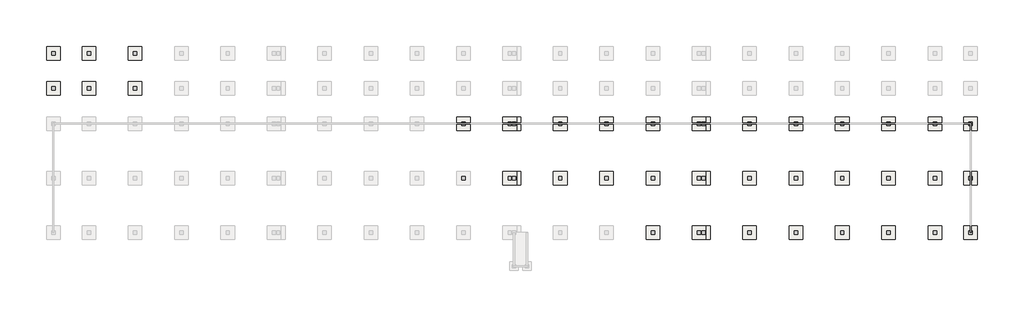
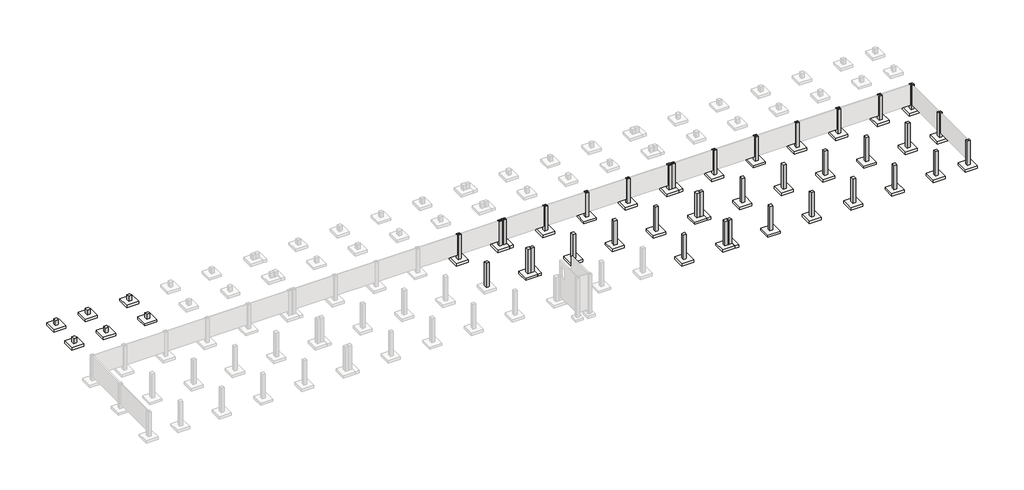
# Not in any storey, part 2 of 3: 43 columns, 42 slabs.
"""IFC4 building model written with IfcOpenShell, lengths in millimetres."""

import ifcopenshell
import ifcopenshell.guid

model = None  # the IFC model being written
_history = None  # IfcOwnerHistory: only IFC2X3 demands one
_inside = {}  # id of a spatial element -> (the spatial element, [elements in it])
_under = {}  # id of a project, library or spatial element -> (it, [spatial elements below it])
_declared = {}  # id of a project -> (the project, [libraries it declares])
_typed = {}  # id of a type object -> (the type object, [elements of that type])
_made_of = {}  # id of a material, layer set ... -> (it, [elements and type objects made of it])


def new_model(schema):
    """Start an empty IFC model of exactly this schema.

    Asked for "IFC4X3", IfcOpenShell would pick the latest addendum, in which some entities
    have other attributes; the version numbers below select the first issue.
    IFC2X3 requires an IfcOwnerHistory on every rooted entity: one is made here for all.
    """
    global model, _history
    if schema == "IFC4X3":
        model = ifcopenshell.file(schema_version=(4, 3, 0, 0))
    else:
        model = ifcopenshell.file(schema=schema)
    _inside.clear()
    _under.clear()
    _declared.clear()
    _typed.clear()
    _made_of.clear()
    _history = None
    if model.schema == "IFC2X3":
        org = make("IfcOrganization", Name="unknown")
        user = make(
            "IfcPersonAndOrganization",
            ThePerson=make("IfcPerson", FamilyName="unknown"),
            TheOrganization=org,
        )
        app = make(
            "IfcApplication",
            ApplicationDeveloper=org,
            Version="unknown",
            ApplicationFullName="unknown",
            ApplicationIdentifier="unknown",
        )
        _history = make(
            "IfcOwnerHistory",
            OwningUser=user,
            OwningApplication=app,
            ChangeAction="ADDED",
            CreationDate=0,
        )
    return model


def make(cls, **values):
    """One entity of the class cls with the attributes given. An attribute that is None is left unset."""
    return model.create_entity(
        cls, **{name: value for name, value in values.items() if value is not None}
    )


def rooted(cls, **values):
    """An entity with a GlobalId (a new one), such as an element, a storey or a relation."""
    return make(cls, GlobalId=ifcopenshell.guid.new(), OwnerHistory=_history, **values)


def si_unit(unit_type, name, prefix=None):
    """IfcSIUnit, for example si_unit("LENGTHUNIT", "METRE", prefix="MILLI")."""
    return make("IfcSIUnit", UnitType=unit_type, Prefix=prefix, Name=name)


def assignment(units):
    """IfcUnitAssignment: the units of a project."""
    return None if units is None else make("IfcUnitAssignment", Units=units)


def point(xyz):
    """IfcCartesianPoint."""
    return None if xyz is None else make("IfcCartesianPoint", Coordinates=xyz)


def direction(xyz):
    """IfcDirection."""
    return None if xyz is None else make("IfcDirection", DirectionRatios=xyz)


def frame(location, z_axis=None, x_axis=None):
    """IfcAxis2Placement3D, a coordinate frame: its origin and axes. An axis left out is left unset."""
    return make(
        "IfcAxis2Placement3D",
        Location=point(location),
        Axis=direction(z_axis),
        RefDirection=direction(x_axis),
    )


def origin():
    """The frame at (0, 0, 0) with its axes left unset."""
    return frame((0.0, 0.0, 0.0))


def place(relative_to, where):
    """IfcLocalPlacement: puts the frame where relative to a parent placement (None: the world)."""
    return make(
        "IfcLocalPlacement", PlacementRelTo=relative_to, RelativePlacement=where
    )


def context(
    kind, dimensions, precision=None, world=None, true_north=None, identifier=None
):
    """IfcGeometricRepresentationContext, for example the 3D "Model" context."""
    return make(
        "IfcGeometricRepresentationContext",
        ContextIdentifier=identifier,
        ContextType=kind,
        CoordinateSpaceDimension=dimensions,
        Precision=precision,
        WorldCoordinateSystem=world,
        TrueNorth=true_north,
    )


def project(units=None, contexts=None):
    """IfcProject with its units and contexts."""
    return rooted(
        "IfcProject",
        Name="project",
        RepresentationContexts=contexts,
        UnitsInContext=assignment(units),
    )


def spatial(cls, under=None, at=None, **own):
    """A site, building, storey or space (cls), placed at a placement, below another one or the project."""
    s = rooted(cls, ObjectPlacement=at, **own)
    if under is not None:
        _under.setdefault(under.id(), (under, []))[1].append(s)
    return s


def polyline(points):
    """IfcPolyline through the points."""
    return make("IfcPolyline", Points=[point(p) for p in points])


def outline(outer, holes=None, kind="AREA"):
    """IfcArbitraryClosedProfileDef: a profile drawn as a closed curve; with holes, ...WithVoids."""
    if holes is None:
        return make("IfcArbitraryClosedProfileDef", ProfileType=kind, OuterCurve=outer)
    return make(
        "IfcArbitraryProfileDefWithVoids",
        ProfileType=kind,
        OuterCurve=outer,
        InnerCurves=holes,
    )


def extrude(swept, where, along, depth):
    """IfcExtrudedAreaSolid: the profile swept, set in the frame where, extruded along a direction by depth."""
    return make(
        "IfcExtrudedAreaSolid",
        SweptArea=swept,
        Position=where,
        ExtrudedDirection=direction(along),
        Depth=depth,
    )


def shape(context_of_items, identifier, shape_type, items):
    """IfcShapeRepresentation: the items that make up one representation, for example the "Body"."""
    return make(
        "IfcShapeRepresentation",
        ContextOfItems=context_of_items,
        RepresentationIdentifier=identifier,
        RepresentationType=shape_type,
        Items=items,
    )


def source(mapping_origin, context_of_items, identifier, shape_type, items):
    """IfcRepresentationMap: a shape defined once, which mapped items show again and again."""
    return make(
        "IfcRepresentationMap",
        MappingOrigin=mapping_origin,
        MappedRepresentation=shape(context_of_items, identifier, shape_type, items),
    )


def transform(
    local_origin,
    x_axis=None,
    y_axis=None,
    z_axis=None,
    scale=None,
    scale2=None,
    scale3=None,
    uniform=True,
):
    """IfcCartesianTransformationOperator3D, or its non-uniform kind. x_axis, y_axis, z_axis: its Axis1, 2, 3."""
    if uniform:
        return make(
            "IfcCartesianTransformationOperator3D",
            Axis1=direction(x_axis),
            Axis2=direction(y_axis),
            LocalOrigin=point(local_origin),
            Scale=scale,
            Axis3=direction(z_axis),
        )
    return make(
        "IfcCartesianTransformationOperator3DnonUniform",
        Axis1=direction(x_axis),
        Axis2=direction(y_axis),
        LocalOrigin=point(local_origin),
        Scale=scale,
        Axis3=direction(z_axis),
        Scale2=scale2,
        Scale3=scale3,
    )


def mapped(mapping_source, mapping_target):
    """IfcMappedItem: shows the shape of a source again, moved by a transform."""
    return make(
        "IfcMappedItem", MappingSource=mapping_source, MappingTarget=mapping_target
    )


def made_of(thing, what):
    """Note that an element or type object is made of a material, layer set ...; save() writes the relation."""
    if what is not None:
        _made_of.setdefault(what.id(), (what, []))[1].append(thing)
    return thing


def element(
    cls,
    number,
    at=None,
    inside=None,
    cuts=None,
    type_object=None,
    material=None,
    context=None,
    identifier="Body",
    shape_type=None,
    held_by="IfcProductDefinitionShape",
    body=None,
    shapes=None,
    **own,
):
    """One element of the class cls, such as IfcWall. Its Tag is "e" and its number.

    at: its placement. inside: the storey or other place that contains it. cuts: it is an
    opening in that element (IfcRelVoidsElement). A single representation is given by context,
    identifier, shape_type and body (its items); several are given by shapes. held_by: the class
    of the entity that holds the representations. save() writes the other relations.
    """
    e = rooted(cls, Tag="e%d" % number, ObjectPlacement=at, **own)
    if body is not None:
        shapes = [shape(context, identifier, shape_type, body)]
    if shapes is not None:
        e.Representation = make(held_by, Representations=shapes)
    if inside is not None:
        _inside.setdefault(inside.id(), (inside, []))[1].append(e)
    if cuts is not None:
        rooted(
            "IfcRelVoidsElement", RelatingBuildingElement=cuts, RelatedOpeningElement=e
        )
    if type_object is not None:
        _typed.setdefault(type_object.id(), (type_object, []))[1].append(e)
    return made_of(e, material)


def aggregate(whole, parts):
    """IfcRelAggregates: a whole, such as a stair, and the parts it consists of."""
    return rooted("IfcRelAggregates", RelatingObject=whole, RelatedObjects=parts)


def save(model, path):
    """Write the relations noted so far, then the file.

    IfcRelAggregates (storeys below a building ...), IfcRelContainedInSpatialStructure (elements
    in a storey), IfcRelDefinesByType, IfcRelAssociatesMaterial and IfcRelDeclares: one each for
    every whole, place, type object, material and project.
    """
    for whole, parts in _under.values():
        aggregate(whole, parts)
    for where, things in _inside.values():
        rooted(
            "IfcRelContainedInSpatialStructure",
            RelatedElements=things,
            RelatingStructure=where,
        )
    for kind, things in _typed.values():
        rooted("IfcRelDefinesByType", RelatedObjects=things, RelatingType=kind)
    for what, things in _made_of.values():
        rooted("IfcRelAssociatesMaterial", RelatedObjects=things, RelatingMaterial=what)
    for by, libraries in _declared.values():
        rooted("IfcRelDeclares", RelatingContext=by, RelatedDefinitions=libraries)
    model.write(path)


def foundation_rectangular_non_pile_5fe39465(model_context):
    return source(origin(), model_context, "Body", "SweptSolid", [
        extrude(outline(polyline([(1200.0, 1200.0), (1200.0, -1200.0), (-1200.0, -1200.0), (-1200.0, 1200.0), (1200.0, 1200.0)])), frame((0.0, 0.0, -500.0), z_axis=(0.0, 0.0, 1.0), x_axis=(1.0, 0.0, 0.0)), (0.0, 0.0, 1.0), 500.0),
    ])


model = new_model("IFC4")

# Units and contexts
model_context = context("Model", 3, world=origin())
ifc_project = project(units=[si_unit("LENGTHUNIT", "METRE", prefix="MILLI")], contexts=[model_context])

# Site, building
site = spatial("IfcSite", under=ifc_project)
building = spatial("IfcBuilding", under=site)

# Columns
placement = place(None, origin())
element("IfcColumn", 1, ObjectType="RC_Column_Rectangular : H_SC_AR_S15_UG PED_W600xL600_Bit_Anchor", at=placement, inside=building, context=model_context, shape_type="SweptSolid", body=[
    extrude(outline(polyline([(-4070.0, 549.5208589), (-4070.0, -50.4791411), (-4670.0, -50.4791411), (-4670.0, 549.5208589), (-4070.0, 549.5208589)])), frame((0.0, 0.0, -750.0381366), z_axis=(0.0, 0.0, 1.0), x_axis=(1.0, 0.0, 0.0)), (0.0, 0.0, 1.0), 1050.0),
])
element("IfcColumn", 2, ObjectType="RC_Column_Rectangular : H_SC_AR_S15_UG PED_W600xL600_Bit_Anchor", at=placement, inside=building, context=model_context, shape_type="SweptSolid", body=[
    extrude(outline(polyline([(2230.0, 549.5208589), (2230.0, -50.4791411), (1630.0, -50.4791411), (1630.0, 549.5208589), (2230.0, 549.5208589)])), frame((0.0, 0.0, -750.0381366), z_axis=(0.0, 0.0, 1.0), x_axis=(1.0, 0.0, 0.0)), (0.0, 0.0, 1.0), 1050.0),
])
element("IfcColumn", 3, ObjectType="RC_Column_Rectangular : H_SC_AR_S15_UG PED_W600xL600_Bit_Anchor", at=placement, inside=building, context=model_context, shape_type="SweptSolid", body=[
    extrude(outline(polyline([(10430.0, 549.5208589), (10430.0, -50.4791411), (9830.0, -50.4791411), (9830.0, 549.5208589), (10430.0, 549.5208589)])), frame((0.0, 0.0, -750.0381366), z_axis=(0.0, 0.0, 1.0), x_axis=(1.0, 0.0, 0.0)), (0.0, 0.0, 1.0), 1050.0),
])
element("IfcColumn", 4, ObjectType="RC_Column_Rectangular : H_SC_AR_S15_UG PED_W600xL600_Bit_Anchor", at=placement, inside=building, context=model_context, shape_type="SweptSolid", body=[
    extrude(outline(polyline([(-4070.0, 6799.5208589), (-4070.0, 6199.5208589), (-4670.0, 6199.5208589), (-4670.0, 6799.5208589), (-4070.0, 6799.5208589)])), frame((0.0, 0.0, -750.0381366), z_axis=(0.0, 0.0, 1.0), x_axis=(1.0, 0.0, 0.0)), (0.0, 0.0, 1.0), 1050.0),
])
element("IfcColumn", 5, ObjectType="RC_Column_Rectangular : H_SC_AR_S15_UG PED_W600xL600_Bit_Anchor", at=placement, inside=building, context=model_context, shape_type="SweptSolid", body=[
    extrude(outline(polyline([(2230.0, 6799.5208589), (2230.0, 6199.5208589), (1630.0, 6199.5208589), (1630.0, 6799.5208589), (2230.0, 6799.5208589)])), frame((0.0, 0.0, -750.0381366), z_axis=(0.0, 0.0, 1.0), x_axis=(1.0, 0.0, 0.0)), (0.0, 0.0, 1.0), 1050.0),
])
element("IfcColumn", 6, ObjectType="RC_Column_Rectangular : H_SC_AR_S15_UG PED_W600xL600_Bit_Anchor", at=placement, inside=building, context=model_context, shape_type="SweptSolid", body=[
    extrude(outline(polyline([(10430.0, 6799.5208589), (10430.0, 6199.5208589), (9830.0, 6199.5208589), (9830.0, 6799.5208589), (10430.0, 6799.5208589)])), frame((0.0, 0.0, -750.0381366), z_axis=(0.0, 0.0, 1.0), x_axis=(1.0, 0.0, 0.0)), (0.0, 0.0, 1.0), 1050.0),
])
element("IfcColumn", 7, ObjectType="RC_Column_Rectangular : H_SC_AR_S15_UG PED_W600xL600_Bit_Anchor", at=placement, inside=building, context=model_context, shape_type="SweptSolid", body=[
    extrude(outline(polyline([(68580.0, -5700.4791411), (68580.0, -6300.4791411), (67980.0, -6300.4791411), (67980.0, -5700.4791411), (68580.0, -5700.4791411)])), frame((0.0, 0.0, -4800.0381366), z_axis=(0.0, 0.0, 1.0), x_axis=(1.0, 0.0, 0.0)), (0.0, 0.0, 1.0), 5100.0),
])
element("IfcColumn", 8, ObjectType="RC_Column_Rectangular : H_SC_AR_S15_UG PED_W600xL600_Bit_Anchor", at=placement, inside=building, context=model_context, shape_type="SweptSolid", body=[
    extrude(outline(polyline([(76780.0, -5700.4791411), (76780.0, -6300.4791411), (76180.0, -6300.4791411), (76180.0, -5700.4791411), (76780.0, -5700.4791411)])), frame((0.0, 0.0, -4800.0381366), z_axis=(0.0, 0.0, 1.0), x_axis=(1.0, 0.0, 0.0)), (0.0, 0.0, 1.0), 5100.0),
])
element("IfcColumn", 9, ObjectType="RC_Column_Rectangular : H_SC_AR_S15_UG PED_W600xL600_Bit_Anchor", at=placement, inside=building, context=model_context, shape_type="SweptSolid", body=[
    extrude(outline(polyline([(77530.0, -5700.4791411), (77530.0, -6300.4791411), (76930.0, -6300.4791411), (76930.0, -5700.4791411), (77530.0, -5700.4791411)])), frame((0.0, 0.0, -4800.0381366), z_axis=(0.0, 0.0, 1.0), x_axis=(1.0, 0.0, 0.0)), (0.0, 0.0, 1.0), 5100.0),
])
element("IfcColumn", 10, ObjectType="RC_Column_Rectangular : H_SC_AR_S15_UG PED_W600xL600_Bit_Anchor", at=placement, inside=building, context=model_context, shape_type="SweptSolid", body=[
    extrude(outline(polyline([(85730.0, -5700.4791411), (85730.0, -6300.4791411), (85130.0, -6300.4791411), (85130.0, -5700.4791411), (85730.0, -5700.4791411)])), frame((0.0, 0.0, -4800.0381366), z_axis=(0.0, 0.0, 1.0), x_axis=(1.0, 0.0, 0.0)), (0.0, 0.0, 1.0), 5100.0),
])
element("IfcColumn", 11, ObjectType="RC_Column_Rectangular : H_SC_AR_S15_UG PED_W600xL600_Bit_Anchor", at=placement, inside=building, context=model_context, shape_type="SweptSolid", body=[
    extrude(outline(polyline([(93930.0, -5700.4791411), (93930.0, -6300.4791411), (93330.0, -6300.4791411), (93330.0, -5700.4791411), (93930.0, -5700.4791411)])), frame((0.0, 0.0, -4800.0381366), z_axis=(0.0, 0.0, 1.0), x_axis=(1.0, 0.0, 0.0)), (0.0, 0.0, 1.0), 5100.0),
])
element("IfcColumn", 12, ObjectType="RC_Column_Rectangular : H_SC_AR_S15_UG PED_W600xL600_Bit_Anchor", at=placement, inside=building, context=model_context, shape_type="SweptSolid", body=[
    extrude(outline(polyline([(102130.0, -5700.4791411), (102130.0, -6300.4791411), (101530.0, -6300.4791411), (101530.0, -5700.4791411), (102130.0, -5700.4791411)])), frame((0.0, 0.0, -4800.0381366), z_axis=(0.0, 0.0, 1.0), x_axis=(1.0, 0.0, 0.0)), (0.0, 0.0, 1.0), 5100.0),
])
element("IfcColumn", 13, ObjectType="RC_Column_Rectangular : H_SC_AR_S15_UG PED_W600xL600_Bit_Anchor", at=placement, inside=building, context=model_context, shape_type="SweptSolid", body=[
    extrude(outline(polyline([(110330.0, -5700.4791411), (110330.0, -6300.4791411), (109730.0, -6300.4791411), (109730.0, -5700.4791411), (110330.0, -5700.4791411)])), frame((0.0, 0.0, -4800.0381366), z_axis=(0.0, 0.0, 1.0), x_axis=(1.0, 0.0, 0.0)), (0.0, 0.0, 1.0), 5100.0),
])
element("IfcColumn", 14, ObjectType="RC_Column_Rectangular : H_SC_AR_S15_UG PED_W600xL600_Bit_Anchor", at=placement, inside=building, context=model_context, shape_type="SweptSolid", body=[
    extrude(outline(polyline([(111080.0, -5700.4791411), (111080.0, -6300.4791411), (110480.0, -6300.4791411), (110480.0, -5700.4791411), (111080.0, -5700.4791411)])), frame((0.0, 0.0, -4800.0381366), z_axis=(0.0, 0.0, 1.0), x_axis=(1.0, 0.0, 0.0)), (0.0, 0.0, 1.0), 5100.0),
])
element("IfcColumn", 15, ObjectType="RC_Column_Rectangular : H_SC_AR_S15_UG PED_W600xL600_Bit_Anchor", at=placement, inside=building, context=model_context, shape_type="SweptSolid", body=[
    extrude(outline(polyline([(119280.0, -5700.4791411), (119280.0, -6300.4791411), (118680.0, -6300.4791411), (118680.0, -5700.4791411), (119280.0, -5700.4791411)])), frame((0.0, 0.0, -4800.0381366), z_axis=(0.0, 0.0, 1.0), x_axis=(1.0, 0.0, 0.0)), (0.0, 0.0, 1.0), 5100.0),
])
element("IfcColumn", 16, ObjectType="RC_Column_Rectangular : H_SC_AR_S15_UG PED_W600xL600_Bit_Anchor", at=placement, inside=building, context=model_context, shape_type="SweptSolid", body=[
    extrude(outline(polyline([(127480.0, -5700.4791411), (127480.0, -6300.4791411), (126880.0, -6300.4791411), (126880.0, -5700.4791411), (127480.0, -5700.4791411)])), frame((0.0, 0.0, -4800.0381366), z_axis=(0.0, 0.0, 1.0), x_axis=(1.0, 0.0, 0.0)), (0.0, 0.0, 1.0), 5100.0),
])
element("IfcColumn", 17, ObjectType="RC_Column_Rectangular : H_SC_AR_S15_UG PED_W600xL600_Bit_Anchor", at=placement, inside=building, context=model_context, shape_type="SweptSolid", body=[
    extrude(outline(polyline([(135680.0, -5700.4791411), (135680.0, -6300.4791411), (135080.0, -6300.4791411), (135080.0, -5700.4791411), (135680.0, -5700.4791411)])), frame((0.0, 0.0, -4800.0381366), z_axis=(0.0, 0.0, 1.0), x_axis=(1.0, 0.0, 0.0)), (0.0, 0.0, 1.0), 5100.0),
])
element("IfcColumn", 18, ObjectType="RC_Column_Rectangular : H_SC_AR_S15_UG PED_W600xL600_Bit_Anchor", at=placement, inside=building, context=model_context, shape_type="SweptSolid", body=[
    extrude(outline(polyline([(143880.0, -5700.4791411), (143880.0, -6300.4791411), (143280.0, -6300.4791411), (143280.0, -5700.4791411), (143880.0, -5700.4791411)])), frame((0.0, 0.0, -4800.0381366), z_axis=(0.0, 0.0, 1.0), x_axis=(1.0, 0.0, 0.0)), (0.0, 0.0, 1.0), 5100.0),
])
element("IfcColumn", 19, ObjectType="RC_Column_Rectangular : H_SC_AR_S15_UG PED_W600xL600_Bit_Anchor", at=placement, inside=building, context=model_context, shape_type="SweptSolid", body=[
    extrude(outline(polyline([(152080.0, -5700.4791411), (152080.0, -6300.4791411), (151480.0, -6300.4791411), (151480.0, -5700.4791411), (152080.0, -5700.4791411)])), frame((0.0, 0.0, -4800.0381366), z_axis=(0.0, 0.0, 1.0), x_axis=(1.0, 0.0, 0.0)), (0.0, 0.0, 1.0), 5100.0),
])
element("IfcColumn", 20, ObjectType="RC_Column_Rectangular : H_SC_AR_S15_UG PED_W600xL600_Bit_Anchor", at=placement, inside=building, context=model_context, shape_type="SweptSolid", body=[
    extrude(outline(polyline([(158430.0, -5700.4791411), (158430.0, -6300.4791411), (157830.0, -6300.4791411), (157830.0, -5700.4791411), (158430.0, -5700.4791411)])), frame((0.0, 0.0, -4800.0381366), z_axis=(0.0, 0.0, 1.0), x_axis=(1.0, 0.0, 0.0)), (0.0, 0.0, 1.0), 5100.0),
])
element("IfcColumn", 21, ObjectType="RC_Column_Rectangular : H_SC_AR_S15_UG PED_W600xL600_Bit_Anchor", at=placement, inside=building, context=model_context, shape_type="SweptSolid", body=[
    extrude(outline(polyline([(68580.0, -15350.4791411), (68580.0, -15950.4791411), (67980.0, -15950.4791411), (67980.0, -15350.4791411), (68580.0, -15350.4791411)])), frame((0.0, 0.0, -4800.0381366), z_axis=(0.0, 0.0, 1.0), x_axis=(1.0, 0.0, 0.0)), (0.0, 0.0, 1.0), 5100.0),
])
element("IfcColumn", 22, ObjectType="RC_Column_Rectangular : H_SC_AR_S15_UG PED_W600xL600_Bit_Anchor", at=placement, inside=building, context=model_context, shape_type="SweptSolid", body=[
    extrude(outline(polyline([(76780.0, -15350.4791411), (76780.0, -15950.4791411), (76180.0, -15950.4791411), (76180.0, -15350.4791411), (76780.0, -15350.4791411)])), frame((0.0, 0.0, -4800.0381366), z_axis=(0.0, 0.0, 1.0), x_axis=(1.0, 0.0, 0.0)), (0.0, 0.0, 1.0), 5100.0),
])
element("IfcColumn", 23, ObjectType="RC_Column_Rectangular : H_SC_AR_S15_UG PED_W600xL600_Bit_Anchor", at=placement, inside=building, context=model_context, shape_type="SweptSolid", body=[
    extrude(outline(polyline([(77530.0, -15350.4791411), (77530.0, -15950.4791411), (76930.0, -15950.4791411), (76930.0, -15350.4791411), (77530.0, -15350.4791411)])), frame((0.0, 0.0, -4800.0381366), z_axis=(0.0, 0.0, 1.0), x_axis=(1.0, 0.0, 0.0)), (0.0, 0.0, 1.0), 5100.0),
])
element("IfcColumn", 24, ObjectType="RC_Column_Rectangular : H_SC_AR_S15_UG PED_W600xL600_Bit_Anchor", at=placement, inside=building, context=model_context, shape_type="SweptSolid", body=[
    extrude(outline(polyline([(85730.0, -15350.4791411), (85730.0, -15950.4791411), (85130.0, -15950.4791411), (85130.0, -15350.4791411), (85730.0, -15350.4791411)])), frame((0.0, 0.0, -4800.0381366), z_axis=(0.0, 0.0, 1.0), x_axis=(1.0, 0.0, 0.0)), (0.0, 0.0, 1.0), 5100.0),
])
element("IfcColumn", 25, ObjectType="RC_Column_Rectangular : H_SC_AR_S15_UG PED_W600xL600_Bit_Anchor", at=placement, inside=building, context=model_context, shape_type="SweptSolid", body=[
    extrude(outline(polyline([(93930.0, -15350.4791411), (93930.0, -15950.4791411), (93330.0, -15950.4791411), (93330.0, -15350.4791411), (93930.0, -15350.4791411)])), frame((0.0, 0.0, -4800.0381366), z_axis=(0.0, 0.0, 1.0), x_axis=(1.0, 0.0, 0.0)), (0.0, 0.0, 1.0), 5100.0),
])
element("IfcColumn", 26, ObjectType="RC_Column_Rectangular : H_SC_AR_S15_UG PED_W600xL600_Bit_Anchor", at=placement, inside=building, context=model_context, shape_type="SweptSolid", body=[
    extrude(outline(polyline([(102130.0, -15350.4791411), (102130.0, -15950.4791411), (101530.0, -15950.4791411), (101530.0, -15350.4791411), (102130.0, -15350.4791411)])), frame((0.0, 0.0, -4800.0381366), z_axis=(0.0, 0.0, 1.0), x_axis=(1.0, 0.0, 0.0)), (0.0, 0.0, 1.0), 5100.0),
])
element("IfcColumn", 27, ObjectType="RC_Column_Rectangular : H_SC_AR_S15_UG PED_W600xL600_Bit_Anchor", at=placement, inside=building, context=model_context, shape_type="SweptSolid", body=[
    extrude(outline(polyline([(110330.0, -15350.4791411), (110330.0, -15950.4791411), (109730.0, -15950.4791411), (109730.0, -15350.4791411), (110330.0, -15350.4791411)])), frame((0.0, 0.0, -4800.0381366), z_axis=(0.0, 0.0, 1.0), x_axis=(1.0, 0.0, 0.0)), (0.0, 0.0, 1.0), 5100.0),
])
element("IfcColumn", 28, ObjectType="RC_Column_Rectangular : H_SC_AR_S15_UG PED_W600xL600_Bit_Anchor", at=placement, inside=building, context=model_context, shape_type="SweptSolid", body=[
    extrude(outline(polyline([(111080.0, -15350.4791411), (111080.0, -15950.4791411), (110480.0, -15950.4791411), (110480.0, -15350.4791411), (111080.0, -15350.4791411)])), frame((0.0, 0.0, -4800.0381366), z_axis=(0.0, 0.0, 1.0), x_axis=(1.0, 0.0, 0.0)), (0.0, 0.0, 1.0), 5100.0),
])
element("IfcColumn", 29, ObjectType="RC_Column_Rectangular : H_SC_AR_S15_UG PED_W600xL600_Bit_Anchor", at=placement, inside=building, context=model_context, shape_type="SweptSolid", body=[
    extrude(outline(polyline([(119280.0, -15350.4791411), (119280.0, -15950.4791411), (118680.0, -15950.4791411), (118680.0, -15350.4791411), (119280.0, -15350.4791411)])), frame((0.0, 0.0, -4800.0381366), z_axis=(0.0, 0.0, 1.0), x_axis=(1.0, 0.0, 0.0)), (0.0, 0.0, 1.0), 5100.0),
])
element("IfcColumn", 30, ObjectType="RC_Column_Rectangular : H_SC_AR_S15_UG PED_W600xL600_Bit_Anchor", at=placement, inside=building, context=model_context, shape_type="SweptSolid", body=[
    extrude(outline(polyline([(127480.0, -15350.4791411), (127480.0, -15950.4791411), (126880.0, -15950.4791411), (126880.0, -15350.4791411), (127480.0, -15350.4791411)])), frame((0.0, 0.0, -4800.0381366), z_axis=(0.0, 0.0, 1.0), x_axis=(1.0, 0.0, 0.0)), (0.0, 0.0, 1.0), 5100.0),
])
element("IfcColumn", 31, ObjectType="RC_Column_Rectangular : H_SC_AR_S15_UG PED_W600xL600_Bit_Anchor", at=placement, inside=building, context=model_context, shape_type="SweptSolid", body=[
    extrude(outline(polyline([(135680.0, -15350.4791411), (135680.0, -15950.4791411), (135080.0, -15950.4791411), (135080.0, -15350.4791411), (135680.0, -15350.4791411)])), frame((0.0, 0.0, -4800.0381366), z_axis=(0.0, 0.0, 1.0), x_axis=(1.0, 0.0, 0.0)), (0.0, 0.0, 1.0), 5100.0),
])
element("IfcColumn", 32, ObjectType="RC_Column_Rectangular : H_SC_AR_S15_UG PED_W600xL600_Bit_Anchor", at=placement, inside=building, context=model_context, shape_type="SweptSolid", body=[
    extrude(outline(polyline([(143880.0, -15350.4791411), (143880.0, -15950.4791411), (143280.0, -15950.4791411), (143280.0, -15350.4791411), (143880.0, -15350.4791411)])), frame((0.0, 0.0, -4800.0381366), z_axis=(0.0, 0.0, 1.0), x_axis=(1.0, 0.0, 0.0)), (0.0, 0.0, 1.0), 5100.0),
])
element("IfcColumn", 33, ObjectType="RC_Column_Rectangular : H_SC_AR_S15_UG PED_W600xL600_Bit_Anchor", at=placement, inside=building, context=model_context, shape_type="SweptSolid", body=[
    extrude(outline(polyline([(152080.0, -15350.4791411), (152080.0, -15950.4791411), (151480.0, -15950.4791411), (151480.0, -15350.4791411), (152080.0, -15350.4791411)])), frame((0.0, 0.0, -4800.0381366), z_axis=(0.0, 0.0, 1.0), x_axis=(1.0, 0.0, 0.0)), (0.0, 0.0, 1.0), 5100.0),
])
element("IfcColumn", 34, ObjectType="RC_Column_Rectangular : H_SC_AR_S15_UG PED_W600xL600_Bit_Anchor", at=placement, inside=building, context=model_context, shape_type="SweptSolid", body=[
    extrude(outline(polyline([(158430.0, -15350.4791411), (158430.0, -15950.4791411), (157830.0, -15950.4791411), (157830.0, -15350.4791411), (158430.0, -15350.4791411)])), frame((0.0, 0.0, -4800.0381366), z_axis=(0.0, 0.0, 1.0), x_axis=(1.0, 0.0, 0.0)), (0.0, 0.0, 1.0), 5100.0),
])
element("IfcColumn", 35, ObjectType="RC_Column_Rectangular : H_SC_AR_S15_UG PED_W600xL600_Bit_Anchor", at=placement, inside=building, context=model_context, shape_type="SweptSolid", body=[
    extrude(outline(polyline([(102130.0, -25000.4791411), (102130.0, -25600.4791411), (101530.0, -25600.4791411), (101530.0, -25000.4791411), (102130.0, -25000.4791411)])), frame((0.0, 0.0, -4800.0381366), z_axis=(0.0, 0.0, 1.0), x_axis=(1.0, 0.0, 0.0)), (0.0, 0.0, 1.0), 5100.0),
])
element("IfcColumn", 36, ObjectType="RC_Column_Rectangular : H_SC_AR_S15_UG PED_W600xL600_Bit_Anchor", at=placement, inside=building, context=model_context, shape_type="SweptSolid", body=[
    extrude(outline(polyline([(110330.0, -25000.4791411), (110330.0, -25600.4791411), (109730.0, -25600.4791411), (109730.0, -25000.4791411), (110330.0, -25000.4791411)])), frame((0.0, 0.0, -4800.0381366), z_axis=(0.0, 0.0, 1.0), x_axis=(1.0, 0.0, 0.0)), (0.0, 0.0, 1.0), 5100.0),
])
element("IfcColumn", 37, ObjectType="RC_Column_Rectangular : H_SC_AR_S15_UG PED_W600xL600_Bit_Anchor", at=placement, inside=building, context=model_context, shape_type="SweptSolid", body=[
    extrude(outline(polyline([(111080.0, -25000.4791411), (111080.0, -25600.4791411), (110480.0, -25600.4791411), (110480.0, -25000.4791411), (111080.0, -25000.4791411)])), frame((0.0, 0.0, -4800.0381366), z_axis=(0.0, 0.0, 1.0), x_axis=(1.0, 0.0, 0.0)), (0.0, 0.0, 1.0), 5100.0),
])
element("IfcColumn", 38, ObjectType="RC_Column_Rectangular : H_SC_AR_S15_UG PED_W600xL600_Bit_Anchor", at=placement, inside=building, context=model_context, shape_type="SweptSolid", body=[
    extrude(outline(polyline([(119280.0, -25000.4791411), (119280.0, -25600.4791411), (118680.0, -25600.4791411), (118680.0, -25000.4791411), (119280.0, -25000.4791411)])), frame((0.0, 0.0, -4800.0381366), z_axis=(0.0, 0.0, 1.0), x_axis=(1.0, 0.0, 0.0)), (0.0, 0.0, 1.0), 5100.0),
])
element("IfcColumn", 39, ObjectType="RC_Column_Rectangular : H_SC_AR_S15_UG PED_W600xL600_Bit_Anchor", at=placement, inside=building, context=model_context, shape_type="SweptSolid", body=[
    extrude(outline(polyline([(127480.0, -25000.4791411), (127480.0, -25600.4791411), (126880.0, -25600.4791411), (126880.0, -25000.4791411), (127480.0, -25000.4791411)])), frame((0.0, 0.0, -4800.0381366), z_axis=(0.0, 0.0, 1.0), x_axis=(1.0, 0.0, 0.0)), (0.0, 0.0, 1.0), 5100.0),
])
element("IfcColumn", 40, ObjectType="RC_Column_Rectangular : H_SC_AR_S15_UG PED_W600xL600_Bit_Anchor", at=placement, inside=building, context=model_context, shape_type="SweptSolid", body=[
    extrude(outline(polyline([(135680.0, -25000.4791411), (135680.0, -25600.4791411), (135080.0, -25600.4791411), (135080.0, -25000.4791411), (135680.0, -25000.4791411)])), frame((0.0, 0.0, -4800.0381366), z_axis=(0.0, 0.0, 1.0), x_axis=(1.0, 0.0, 0.0)), (0.0, 0.0, 1.0), 5100.0),
])
element("IfcColumn", 41, ObjectType="RC_Column_Rectangular : H_SC_AR_S15_UG PED_W600xL600_Bit_Anchor", at=placement, inside=building, context=model_context, shape_type="SweptSolid", body=[
    extrude(outline(polyline([(143880.0, -25000.4791411), (143880.0, -25600.4791411), (143280.0, -25600.4791411), (143280.0, -25000.4791411), (143880.0, -25000.4791411)])), frame((0.0, 0.0, -4800.0381366), z_axis=(0.0, 0.0, 1.0), x_axis=(1.0, 0.0, 0.0)), (0.0, 0.0, 1.0), 5100.0),
])
element("IfcColumn", 42, ObjectType="RC_Column_Rectangular : H_SC_AR_S15_UG PED_W600xL600_Bit_Anchor", at=placement, inside=building, context=model_context, shape_type="SweptSolid", body=[
    extrude(outline(polyline([(152080.0, -25000.4791411), (152080.0, -25600.4791411), (151480.0, -25600.4791411), (151480.0, -25000.4791411), (152080.0, -25000.4791411)])), frame((0.0, 0.0, -4800.0381366), z_axis=(0.0, 0.0, 1.0), x_axis=(1.0, 0.0, 0.0)), (0.0, 0.0, 1.0), 5100.0),
])
element("IfcColumn", 43, ObjectType="RC_Column_Rectangular : H_SC_AR_S15_UG PED_W600xL600_Bit_Anchor", at=placement, inside=building, context=model_context, shape_type="SweptSolid", body=[
    extrude(outline(polyline([(158430.0, -25000.4791411), (158430.0, -25600.4791411), (157830.0, -25600.4791411), (157830.0, -25000.4791411), (158430.0, -25000.4791411)])), frame((0.0, 0.0, -4800.0381366), z_axis=(0.0, 0.0, 1.0), x_axis=(1.0, 0.0, 0.0)), (0.0, 0.0, 1.0), 5100.0),
])

# Slabs
element("IfcSlab", 44, ObjectType="Foundation Rectangular (Non-Pile) : H_SF_AR_S18_W2400xL2400xT500_Bitumen", at=placement, inside=building, context=model_context, shape_type="SweptSolid", body=[
    extrude(outline(polyline([(77680.0, -4800.4791411), (77680.0, -7200.4791411), (75280.0, -7200.4791411), (75280.0, -4800.4791411), (77680.0, -4800.4791411)])), frame((0.0, 0.0, -5300.0381366), z_axis=(0.0, 0.0, 1.0), x_axis=(1.0, 0.0, 0.0)), (0.0, 0.0, 1.0), 500.0),
])
element("IfcSlab", 45, ObjectType="Foundation Rectangular (Non-Pile) : H_SF_AR_S18_W2400xL2400xT500_Bitumen", at=placement, inside=building, context=model_context, shape_type="SweptSolid", body=[
    extrude(outline(polyline([(78430.0, -4800.4791411), (78430.0, -7200.4791411), (77680.0, -7200.4791411), (77680.0, -4800.4791411), (78430.0, -4800.4791411)])), frame((0.0, 0.0, -5300.0381366), z_axis=(0.0, 0.0, 1.0), x_axis=(1.0, 0.0, 0.0)), (0.0, 0.0, 1.0), 500.0),
])
element("IfcSlab", 46, ObjectType="Foundation Rectangular (Non-Pile) : H_SF_AR_S18_W2400xL2400xT500_Bitumen", at=placement, inside=building, context=model_context, shape_type="SweptSolid", body=[
    extrude(outline(polyline([(111230.0, -4800.4791411), (111230.0, -7200.4791411), (108830.0, -7200.4791411), (108830.0, -4800.4791411), (111230.0, -4800.4791411)])), frame((0.0, 0.0, -5300.0381366), z_axis=(0.0, 0.0, 1.0), x_axis=(1.0, 0.0, 0.0)), (0.0, 0.0, 1.0), 500.0),
])
element("IfcSlab", 47, ObjectType="Foundation Rectangular (Non-Pile) : H_SF_AR_S18_W2400xL2400xT500_Bitumen", at=placement, inside=building, context=model_context, shape_type="SweptSolid", body=[
    extrude(outline(polyline([(111980.0, -4800.4791411), (111980.0, -7200.4791411), (111230.0, -7200.4791411), (111230.0, -4800.4791411), (111980.0, -4800.4791411)])), frame((0.0, 0.0, -5300.0381366), z_axis=(0.0, 0.0, 1.0), x_axis=(1.0, 0.0, 0.0)), (0.0, 0.0, 1.0), 500.0),
])
element("IfcSlab", 48, ObjectType="Foundation Rectangular (Non-Pile) : H_SF_AR_S18_W2400xL2400xT500_Bitumen", at=placement, inside=building, context=model_context, shape_type="SweptSolid", body=[
    extrude(outline(polyline([(77680.0, -14450.4791411), (77680.0, -16850.4791411), (75280.0, -16850.4791411), (75280.0, -14450.4791411), (77680.0, -14450.4791411)])), frame((0.0, 0.0, -5300.0381366), z_axis=(0.0, 0.0, 1.0), x_axis=(1.0, 0.0, 0.0)), (0.0, 0.0, 1.0), 500.0),
])
element("IfcSlab", 49, ObjectType="Foundation Rectangular (Non-Pile) : H_SF_AR_S18_W2400xL2400xT500_Bitumen", at=placement, inside=building, context=model_context, shape_type="SweptSolid", body=[
    extrude(outline(polyline([(78430.0, -14450.4791411), (78430.0, -16850.4791411), (77680.0, -16850.4791411), (77680.0, -14450.4791411), (78430.0, -14450.4791411)])), frame((0.0, 0.0, -5300.0381366), z_axis=(0.0, 0.0, 1.0), x_axis=(1.0, 0.0, 0.0)), (0.0, 0.0, 1.0), 500.0),
])
element("IfcSlab", 50, ObjectType="Foundation Rectangular (Non-Pile) : H_SF_AR_S18_W2400xL2400xT500_Bitumen", at=placement, inside=building, context=model_context, shape_type="SweptSolid", body=[
    extrude(outline(polyline([(111230.0, -14450.4791411), (111230.0, -16850.4791411), (108830.0, -16850.4791411), (108830.0, -14450.4791411), (111230.0, -14450.4791411)])), frame((0.0, 0.0, -5300.0381366), z_axis=(0.0, 0.0, 1.0), x_axis=(1.0, 0.0, 0.0)), (0.0, 0.0, 1.0), 500.0),
])
element("IfcSlab", 51, ObjectType="Foundation Rectangular (Non-Pile) : H_SF_AR_S18_W2400xL2400xT500_Bitumen", at=placement, inside=building, context=model_context, shape_type="SweptSolid", body=[
    extrude(outline(polyline([(111980.0, -14450.4791411), (111980.0, -16850.4791411), (111230.0, -16850.4791411), (111230.0, -14450.4791411), (111980.0, -14450.4791411)])), frame((0.0, 0.0, -5300.0381366), z_axis=(0.0, 0.0, 1.0), x_axis=(1.0, 0.0, 0.0)), (0.0, 0.0, 1.0), 500.0),
])
element("IfcSlab", 52, ObjectType="Foundation Rectangular (Non-Pile) : H_SF_AR_S18_W2400xL2400xT500_Bitumen", at=placement, inside=building, context=model_context, shape_type="SweptSolid", body=[
    extrude(outline(polyline([(111230.0, -24100.4791411), (111230.0, -26500.4791411), (108830.0, -26500.4791411), (108830.0, -24100.4791411), (111230.0, -24100.4791411)])), frame((0.0, 0.0, -5300.0381366), z_axis=(0.0, 0.0, 1.0), x_axis=(1.0, 0.0, 0.0)), (0.0, 0.0, 1.0), 500.0),
])
element("IfcSlab", 53, ObjectType="Foundation Rectangular (Non-Pile) : H_SF_AR_S18_W2400xL2400xT500_Bitumen", at=placement, inside=building, context=model_context, shape_type="SweptSolid", body=[
    extrude(outline(polyline([(111980.0, -24100.4791411), (111980.0, -26500.4791411), (111230.0, -26500.4791411), (111230.0, -24100.4791411), (111980.0, -24100.4791411)])), frame((0.0, 0.0, -5300.0381366), z_axis=(0.0, 0.0, 1.0), x_axis=(1.0, 0.0, 0.0)), (0.0, 0.0, 1.0), 500.0),
])
foundation_rectangular_non_pile_shape = foundation_rectangular_non_pile_5fe39465(model_context)
element("IfcSlab", 54, ObjectType="Foundation Rectangular (Non-Pile) : H_SF_AR_S18_W2400xL2400xT500_Bitumen", at=placement, inside=building, context=model_context, shape_type="MappedRepresentation", body=[
    mapped(foundation_rectangular_non_pile_shape, transform((-4370.0, 249.5208589, -750.0381366), x_axis=(1.0, 0.0, 0.0), y_axis=(0.0, 1.0, 0.0), z_axis=(0.0, 0.0, 1.0))),
])
element("IfcSlab", 55, ObjectType="Foundation Rectangular (Non-Pile) : H_SF_AR_S18_W2400xL2400xT500_Bitumen", at=placement, inside=building, context=model_context, shape_type="MappedRepresentation", body=[
    mapped(foundation_rectangular_non_pile_shape, transform((1930.0, 249.5208589, -750.0381366), x_axis=(1.0, 0.0, 0.0), y_axis=(0.0, 1.0, 0.0), z_axis=(0.0, 0.0, 1.0))),
])
element("IfcSlab", 56, ObjectType="Foundation Rectangular (Non-Pile) : H_SF_AR_S18_W2400xL2400xT500_Bitumen", at=placement, inside=building, context=model_context, shape_type="MappedRepresentation", body=[
    mapped(foundation_rectangular_non_pile_shape, transform((10130.0, 249.5208589, -750.0381366), x_axis=(1.0, 0.0, 0.0), y_axis=(0.0, 1.0, 0.0), z_axis=(0.0, 0.0, 1.0))),
])
element("IfcSlab", 57, ObjectType="Foundation Rectangular (Non-Pile) : H_SF_AR_S18_W2400xL2400xT500_Bitumen", at=placement, inside=building, context=model_context, shape_type="MappedRepresentation", body=[
    mapped(foundation_rectangular_non_pile_shape, transform((-4370.0, 6499.5208589, -750.0381366), x_axis=(1.0, 0.0, 0.0), y_axis=(0.0, 1.0, 0.0), z_axis=(0.0, 0.0, 1.0))),
])
element("IfcSlab", 58, ObjectType="Foundation Rectangular (Non-Pile) : H_SF_AR_S18_W2400xL2400xT500_Bitumen", at=placement, inside=building, context=model_context, shape_type="MappedRepresentation", body=[
    mapped(foundation_rectangular_non_pile_shape, transform((1930.0, 6499.5208589, -750.0381366), x_axis=(1.0, 0.0, 0.0), y_axis=(0.0, 1.0, 0.0), z_axis=(0.0, 0.0, 1.0))),
])
element("IfcSlab", 59, ObjectType="Foundation Rectangular (Non-Pile) : H_SF_AR_S18_W2400xL2400xT500_Bitumen", at=placement, inside=building, context=model_context, shape_type="MappedRepresentation", body=[
    mapped(foundation_rectangular_non_pile_shape, transform((10130.0, 6499.5208589, -750.0381366), x_axis=(1.0, 0.0, 0.0), y_axis=(0.0, 1.0, 0.0), z_axis=(0.0, 0.0, 1.0))),
])
element("IfcSlab", 60, ObjectType="Foundation Rectangular (Non-Pile) : H_SF_AR_S18_W2400xL2400xT500_Bitumen", at=placement, inside=building, context=model_context, shape_type="MappedRepresentation", body=[
    mapped(foundation_rectangular_non_pile_shape, transform((68280.0, -6000.4791411, -4800.0381366), x_axis=(1.0, 0.0, 0.0), y_axis=(0.0, 1.0, 0.0), z_axis=(0.0, 0.0, 1.0))),
])
element("IfcSlab", 61, ObjectType="Foundation Rectangular (Non-Pile) : H_SF_AR_S18_W2400xL2400xT500_Bitumen", at=placement, inside=building, context=model_context, shape_type="MappedRepresentation", body=[
    mapped(foundation_rectangular_non_pile_shape, transform((85430.0, -6000.4791411, -4800.0381366), x_axis=(1.0, 0.0, 0.0), y_axis=(0.0, 1.0, 0.0), z_axis=(0.0, 0.0, 1.0))),
])
element("IfcSlab", 62, ObjectType="Foundation Rectangular (Non-Pile) : H_SF_AR_S18_W2400xL2400xT500_Bitumen", at=placement, inside=building, context=model_context, shape_type="MappedRepresentation", body=[
    mapped(foundation_rectangular_non_pile_shape, transform((93630.0, -6000.4791411, -4800.0381366), x_axis=(1.0, 0.0, 0.0), y_axis=(0.0, 1.0, 0.0), z_axis=(0.0, 0.0, 1.0))),
])
element("IfcSlab", 63, ObjectType="Foundation Rectangular (Non-Pile) : H_SF_AR_S18_W2400xL2400xT500_Bitumen", at=placement, inside=building, context=model_context, shape_type="MappedRepresentation", body=[
    mapped(foundation_rectangular_non_pile_shape, transform((101830.0, -6000.4791411, -4800.0381366), x_axis=(1.0, 0.0, 0.0), y_axis=(0.0, 1.0, 0.0), z_axis=(0.0, 0.0, 1.0))),
])
element("IfcSlab", 64, ObjectType="Foundation Rectangular (Non-Pile) : H_SF_AR_S18_W2400xL2400xT500_Bitumen", at=placement, inside=building, context=model_context, shape_type="MappedRepresentation", body=[
    mapped(foundation_rectangular_non_pile_shape, transform((118980.0, -6000.4791411, -4800.0381366), x_axis=(1.0, 0.0, 0.0), y_axis=(0.0, 1.0, 0.0), z_axis=(0.0, 0.0, 1.0))),
])
element("IfcSlab", 65, ObjectType="Foundation Rectangular (Non-Pile) : H_SF_AR_S18_W2400xL2400xT500_Bitumen", at=placement, inside=building, context=model_context, shape_type="MappedRepresentation", body=[
    mapped(foundation_rectangular_non_pile_shape, transform((127180.0, -6000.4791411, -4800.0381366), x_axis=(1.0, 0.0, 0.0), y_axis=(0.0, 1.0, 0.0), z_axis=(0.0, 0.0, 1.0))),
])
element("IfcSlab", 66, ObjectType="Foundation Rectangular (Non-Pile) : H_SF_AR_S18_W2400xL2400xT500_Bitumen", at=placement, inside=building, context=model_context, shape_type="MappedRepresentation", body=[
    mapped(foundation_rectangular_non_pile_shape, transform((135380.0, -6000.4791411, -4800.0381366), x_axis=(1.0, 0.0, 0.0), y_axis=(0.0, 1.0, 0.0), z_axis=(0.0, 0.0, 1.0))),
])
element("IfcSlab", 67, ObjectType="Foundation Rectangular (Non-Pile) : H_SF_AR_S18_W2400xL2400xT500_Bitumen", at=placement, inside=building, context=model_context, shape_type="MappedRepresentation", body=[
    mapped(foundation_rectangular_non_pile_shape, transform((143580.0, -6000.4791411, -4800.0381366), x_axis=(1.0, 0.0, 0.0), y_axis=(0.0, 1.0, 0.0), z_axis=(0.0, 0.0, 1.0))),
])
element("IfcSlab", 68, ObjectType="Foundation Rectangular (Non-Pile) : H_SF_AR_S18_W2400xL2400xT500_Bitumen", at=placement, inside=building, context=model_context, shape_type="MappedRepresentation", body=[
    mapped(foundation_rectangular_non_pile_shape, transform((151780.0, -6000.4791411, -4800.0381366), x_axis=(1.0, 0.0, 0.0), y_axis=(0.0, 1.0, 0.0), z_axis=(0.0, 0.0, 1.0))),
])
element("IfcSlab", 69, ObjectType="Foundation Rectangular (Non-Pile) : H_SF_AR_S18_W2400xL2400xT500_Bitumen", at=placement, inside=building, context=model_context, shape_type="MappedRepresentation", body=[
    mapped(foundation_rectangular_non_pile_shape, transform((158130.0, -6000.4791411, -4800.0381366), x_axis=(1.0, 0.0, 0.0), y_axis=(0.0, 1.0, 0.0), z_axis=(0.0, 0.0, 1.0))),
])
element("IfcSlab", 70, ObjectType="Foundation Rectangular (Non-Pile) : H_SF_AR_S18_W2400xL2400xT500_Bitumen", at=placement, inside=building, context=model_context, shape_type="MappedRepresentation", body=[
    mapped(foundation_rectangular_non_pile_shape, transform((85430.0, -15650.4791411, -4800.0381366), x_axis=(1.0, 0.0, 0.0), y_axis=(0.0, 1.0, 0.0), z_axis=(0.0, 0.0, 1.0))),
])
element("IfcSlab", 71, ObjectType="Foundation Rectangular (Non-Pile) : H_SF_AR_S18_W2400xL2400xT500_Bitumen", at=placement, inside=building, context=model_context, shape_type="MappedRepresentation", body=[
    mapped(foundation_rectangular_non_pile_shape, transform((93630.0, -15650.4791411, -4800.0381366), x_axis=(1.0, 0.0, 0.0), y_axis=(0.0, 1.0, 0.0), z_axis=(0.0, 0.0, 1.0))),
])
element("IfcSlab", 72, ObjectType="Foundation Rectangular (Non-Pile) : H_SF_AR_S18_W2400xL2400xT500_Bitumen", at=placement, inside=building, context=model_context, shape_type="MappedRepresentation", body=[
    mapped(foundation_rectangular_non_pile_shape, transform((101830.0, -15650.4791411, -4800.0381366), x_axis=(1.0, 0.0, 0.0), y_axis=(0.0, 1.0, 0.0), z_axis=(0.0, 0.0, 1.0))),
])
element("IfcSlab", 73, ObjectType="Foundation Rectangular (Non-Pile) : H_SF_AR_S18_W2400xL2400xT500_Bitumen", at=placement, inside=building, context=model_context, shape_type="MappedRepresentation", body=[
    mapped(foundation_rectangular_non_pile_shape, transform((118980.0, -15650.4791411, -4800.0381366), x_axis=(1.0, 0.0, 0.0), y_axis=(0.0, 1.0, 0.0), z_axis=(0.0, 0.0, 1.0))),
])
element("IfcSlab", 74, ObjectType="Foundation Rectangular (Non-Pile) : H_SF_AR_S18_W2400xL2400xT500_Bitumen", at=placement, inside=building, context=model_context, shape_type="MappedRepresentation", body=[
    mapped(foundation_rectangular_non_pile_shape, transform((127180.0, -15650.4791411, -4800.0381366), x_axis=(1.0, 0.0, 0.0), y_axis=(0.0, 1.0, 0.0), z_axis=(0.0, 0.0, 1.0))),
])
element("IfcSlab", 75, ObjectType="Foundation Rectangular (Non-Pile) : H_SF_AR_S18_W2400xL2400xT500_Bitumen", at=placement, inside=building, context=model_context, shape_type="MappedRepresentation", body=[
    mapped(foundation_rectangular_non_pile_shape, transform((135380.0, -15650.4791411, -4800.0381366), x_axis=(1.0, 0.0, 0.0), y_axis=(0.0, 1.0, 0.0), z_axis=(0.0, 0.0, 1.0))),
])
element("IfcSlab", 76, ObjectType="Foundation Rectangular (Non-Pile) : H_SF_AR_S18_W2400xL2400xT500_Bitumen", at=placement, inside=building, context=model_context, shape_type="MappedRepresentation", body=[
    mapped(foundation_rectangular_non_pile_shape, transform((143580.0, -15650.4791411, -4800.0381366), x_axis=(1.0, 0.0, 0.0), y_axis=(0.0, 1.0, 0.0), z_axis=(0.0, 0.0, 1.0))),
])
element("IfcSlab", 77, ObjectType="Foundation Rectangular (Non-Pile) : H_SF_AR_S18_W2400xL2400xT500_Bitumen", at=placement, inside=building, context=model_context, shape_type="MappedRepresentation", body=[
    mapped(foundation_rectangular_non_pile_shape, transform((151780.0, -15650.4791411, -4800.0381366), x_axis=(1.0, 0.0, 0.0), y_axis=(0.0, 1.0, 0.0), z_axis=(0.0, 0.0, 1.0))),
])
element("IfcSlab", 78, ObjectType="Foundation Rectangular (Non-Pile) : H_SF_AR_S18_W2400xL2400xT500_Bitumen", at=placement, inside=building, context=model_context, shape_type="MappedRepresentation", body=[
    mapped(foundation_rectangular_non_pile_shape, transform((158130.0, -15650.4791411, -4800.0381366), x_axis=(1.0, 0.0, 0.0), y_axis=(0.0, 1.0, 0.0), z_axis=(0.0, 0.0, 1.0))),
])
element("IfcSlab", 79, ObjectType="Foundation Rectangular (Non-Pile) : H_SF_AR_S18_W2400xL2400xT500_Bitumen", at=placement, inside=building, context=model_context, shape_type="MappedRepresentation", body=[
    mapped(foundation_rectangular_non_pile_shape, transform((101830.0, -25300.4791411, -4800.0381366), x_axis=(1.0, 0.0, 0.0), y_axis=(0.0, 1.0, 0.0), z_axis=(0.0, 0.0, 1.0))),
])
element("IfcSlab", 80, ObjectType="Foundation Rectangular (Non-Pile) : H_SF_AR_S18_W2400xL2400xT500_Bitumen", at=placement, inside=building, context=model_context, shape_type="MappedRepresentation", body=[
    mapped(foundation_rectangular_non_pile_shape, transform((118980.0, -25300.4791411, -4800.0381366), x_axis=(1.0, 0.0, 0.0), y_axis=(0.0, 1.0, 0.0), z_axis=(0.0, 0.0, 1.0))),
])
element("IfcSlab", 81, ObjectType="Foundation Rectangular (Non-Pile) : H_SF_AR_S18_W2400xL2400xT500_Bitumen", at=placement, inside=building, context=model_context, shape_type="MappedRepresentation", body=[
    mapped(foundation_rectangular_non_pile_shape, transform((127180.0, -25300.4791411, -4800.0381366), x_axis=(1.0, 0.0, 0.0), y_axis=(0.0, 1.0, 0.0), z_axis=(0.0, 0.0, 1.0))),
])
element("IfcSlab", 82, ObjectType="Foundation Rectangular (Non-Pile) : H_SF_AR_S18_W2400xL2400xT500_Bitumen", at=placement, inside=building, context=model_context, shape_type="MappedRepresentation", body=[
    mapped(foundation_rectangular_non_pile_shape, transform((135380.0, -25300.4791411, -4800.0381366), x_axis=(1.0, 0.0, 0.0), y_axis=(0.0, 1.0, 0.0), z_axis=(0.0, 0.0, 1.0))),
])
element("IfcSlab", 83, ObjectType="Foundation Rectangular (Non-Pile) : H_SF_AR_S18_W2400xL2400xT500_Bitumen", at=placement, inside=building, context=model_context, shape_type="MappedRepresentation", body=[
    mapped(foundation_rectangular_non_pile_shape, transform((143580.0, -25300.4791411, -4800.0381366), x_axis=(1.0, 0.0, 0.0), y_axis=(0.0, 1.0, 0.0), z_axis=(0.0, 0.0, 1.0))),
])
element("IfcSlab", 84, ObjectType="Foundation Rectangular (Non-Pile) : H_SF_AR_S18_W2400xL2400xT500_Bitumen", at=placement, inside=building, context=model_context, shape_type="MappedRepresentation", body=[
    mapped(foundation_rectangular_non_pile_shape, transform((151780.0, -25300.4791411, -4800.0381366), x_axis=(1.0, 0.0, 0.0), y_axis=(0.0, 1.0, 0.0), z_axis=(0.0, 0.0, 1.0))),
])
element("IfcSlab", 85, ObjectType="Foundation Rectangular (Non-Pile) : H_SF_AR_S18_W2400xL2400xT500_Bitumen", at=placement, inside=building, context=model_context, shape_type="MappedRepresentation", body=[
    mapped(foundation_rectangular_non_pile_shape, transform((158130.0, -25300.4791411, -4800.0381366), x_axis=(1.0, 0.0, 0.0), y_axis=(0.0, 1.0, 0.0), z_axis=(0.0, 0.0, 1.0))),
])

save(model, "model.ifc")

# Revit data of these elements
# Type "RC_Column_Rectangular : H_SC_AR_S15_UG PED_W600xL600_Bit_Anchor"
#   Width = 600 mm
#   Length = 600 mm
#   hec_material3 [instance default] = none
#   hec_material2 [instance default] = none
#   hec_material1 [instance default] = none
#   Structural Material [instance default] = none
#   Description = (empty or 0)
# Type "Foundation Rectangular (Non-Pile) : H_SF_AR_S18_W2400xL2400xT500_Bitumen"
#   Top bar = "D25@300"
#   Description = "UG Shallow Foundation"
#   Bottom bar = "D20@300"
#   Width = 2400 mm
#   Length = 2400 mm
#   Foundation Thickness = 500 mm
#   Structural Material [instance default] = none
#   Assembly Code = ""
# Elements 1, 2, 3, 4, 5, 6, 7, 8, 9, 10, 11, 12, 13, 14, 15, 16, 17, 18, 19, 20, 21, 22, 23, 24, 25, 26, 27, 28, 29, 30, 31, 32, 33, 34, 35, 36, 37, 38, 39, 40, 41, 42, 43 (IfcColumn, "RC_Column_Rectangular : H_SC_AR_S15_UG PED_W600xL600_Bit_Anchor")
#   Comments = ""
#   hec_material3 = none
#   hec_material2 = none
#   hec_material1 = none
#   Structural Material = none
#   Phase Created = New Construction
# Elements 44, 45, 46, 47, 48, 49, 50, 51, 52, 53, 54, 55, 56, 57, 58, 59, 60, 61, 62, 63, 64, 65, 66, 67, 68, 69, 70, 71, 72, 73, 74, 75, 76, 77, 78, 79, 80, 81, 82, 83, 84, 85 (IfcSlab, "Foundation Rectangular (Non-Pile) : H_SF_AR_S18_W2400xL2400xT500_Bitumen")
#   Comments = ""
#   Structural Material = none
#   Phase Created = New Construction
